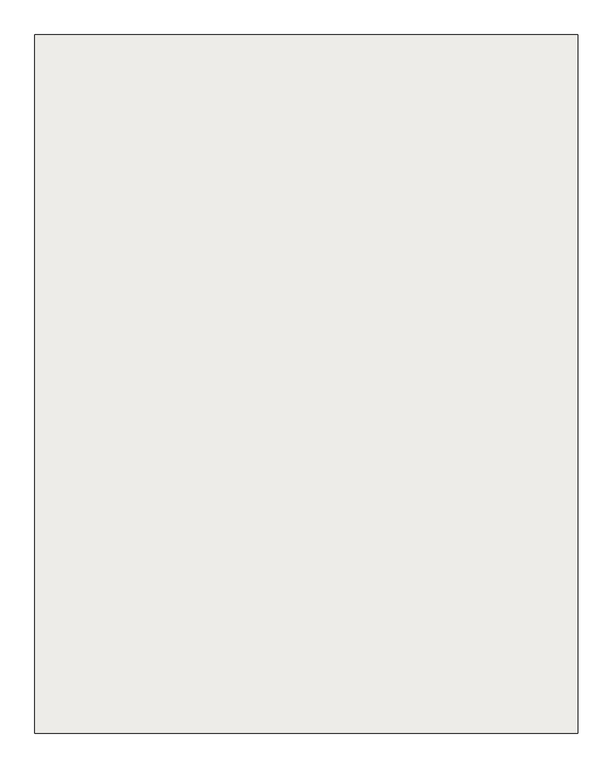
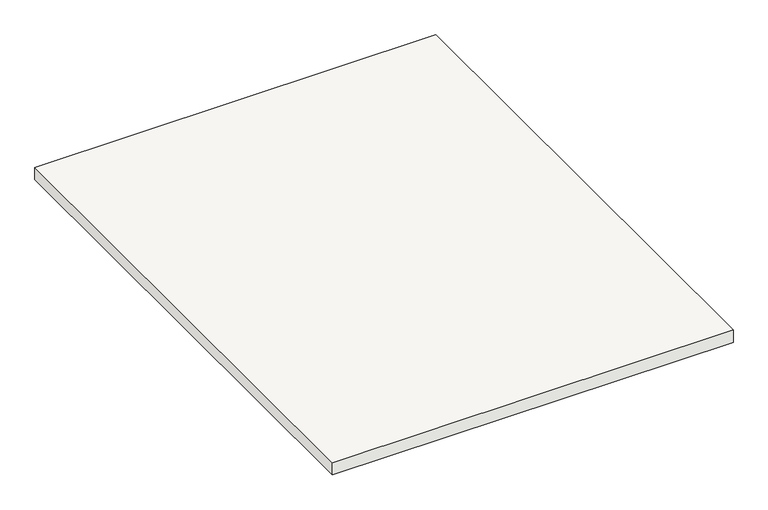
"""IFC4 building model written with IfcOpenShell, lengths in millimetres: slab geometry, Holzdecke 176 : Holzdecke 176."""

import ifcopenshell
import ifcopenshell.guid

model = None  # the IFC model being written
_history = None  # IfcOwnerHistory: only IFC2X3 demands one
_inside = {}  # id of a spatial element -> (the spatial element, [elements in it])
_under = {}  # id of a project, library or spatial element -> (it, [spatial elements below it])
_declared = {}  # id of a project -> (the project, [libraries it declares])
_typed = {}  # id of a type object -> (the type object, [elements of that type])
_made_of = {}  # id of a material, layer set ... -> (it, [elements and type objects made of it])


def new_model(schema):
    """Start an empty IFC model of exactly this schema.

    Asked for "IFC4X3", IfcOpenShell would pick the latest addendum, in which some entities
    have other attributes; the version numbers below select the first issue.
    IFC2X3 requires an IfcOwnerHistory on every rooted entity: one is made here for all.
    """
    global model, _history
    if schema == "IFC4X3":
        model = ifcopenshell.file(schema_version=(4, 3, 0, 0))
    else:
        model = ifcopenshell.file(schema=schema)
    _inside.clear()
    _under.clear()
    _declared.clear()
    _typed.clear()
    _made_of.clear()
    _history = None
    if model.schema == "IFC2X3":
        org = make("IfcOrganization", Name="unknown")
        user = make(
            "IfcPersonAndOrganization",
            ThePerson=make("IfcPerson", FamilyName="unknown"),
            TheOrganization=org,
        )
        app = make(
            "IfcApplication",
            ApplicationDeveloper=org,
            Version="unknown",
            ApplicationFullName="unknown",
            ApplicationIdentifier="unknown",
        )
        _history = make(
            "IfcOwnerHistory",
            OwningUser=user,
            OwningApplication=app,
            ChangeAction="ADDED",
            CreationDate=0,
        )
    return model


def make(cls, **values):
    """One entity of the class cls with the attributes given. An attribute that is None is left unset."""
    return model.create_entity(
        cls, **{name: value for name, value in values.items() if value is not None}
    )


def rooted(cls, **values):
    """An entity with a GlobalId (a new one), such as an element, a storey or a relation."""
    return make(cls, GlobalId=ifcopenshell.guid.new(), OwnerHistory=_history, **values)


def si_unit(unit_type, name, prefix=None):
    """IfcSIUnit, for example si_unit("LENGTHUNIT", "METRE", prefix="MILLI")."""
    return make("IfcSIUnit", UnitType=unit_type, Prefix=prefix, Name=name)


def assignment(units):
    """IfcUnitAssignment: the units of a project."""
    return None if units is None else make("IfcUnitAssignment", Units=units)


def point(xyz):
    """IfcCartesianPoint."""
    return None if xyz is None else make("IfcCartesianPoint", Coordinates=xyz)


def direction(xyz):
    """IfcDirection."""
    return None if xyz is None else make("IfcDirection", DirectionRatios=xyz)


def frame(location, z_axis=None, x_axis=None):
    """IfcAxis2Placement3D, a coordinate frame: its origin and axes. An axis left out is left unset."""
    return make(
        "IfcAxis2Placement3D",
        Location=point(location),
        Axis=direction(z_axis),
        RefDirection=direction(x_axis),
    )


def origin():
    """The frame at (0, 0, 0) with its axes left unset."""
    return frame((0.0, 0.0, 0.0))


def place(relative_to, where):
    """IfcLocalPlacement: puts the frame where relative to a parent placement (None: the world)."""
    return make(
        "IfcLocalPlacement", PlacementRelTo=relative_to, RelativePlacement=where
    )


def context(
    kind, dimensions, precision=None, world=None, true_north=None, identifier=None
):
    """IfcGeometricRepresentationContext, for example the 3D "Model" context."""
    return make(
        "IfcGeometricRepresentationContext",
        ContextIdentifier=identifier,
        ContextType=kind,
        CoordinateSpaceDimension=dimensions,
        Precision=precision,
        WorldCoordinateSystem=world,
        TrueNorth=true_north,
    )


def project(units=None, contexts=None):
    """IfcProject with its units and contexts."""
    return rooted(
        "IfcProject",
        Name="project",
        RepresentationContexts=contexts,
        UnitsInContext=assignment(units),
    )


def spatial(cls, under=None, at=None, **own):
    """A site, building, storey or space (cls), placed at a placement, below another one or the project."""
    s = rooted(cls, ObjectPlacement=at, **own)
    if under is not None:
        _under.setdefault(under.id(), (under, []))[1].append(s)
    return s


def polyline(points):
    """IfcPolyline through the points."""
    return make("IfcPolyline", Points=[point(p) for p in points])


def outline(outer, holes=None, kind="AREA"):
    """IfcArbitraryClosedProfileDef: a profile drawn as a closed curve; with holes, ...WithVoids."""
    if holes is None:
        return make("IfcArbitraryClosedProfileDef", ProfileType=kind, OuterCurve=outer)
    return make(
        "IfcArbitraryProfileDefWithVoids",
        ProfileType=kind,
        OuterCurve=outer,
        InnerCurves=holes,
    )


def extrude(swept, where, along, depth):
    """IfcExtrudedAreaSolid: the profile swept, set in the frame where, extruded along a direction by depth."""
    return make(
        "IfcExtrudedAreaSolid",
        SweptArea=swept,
        Position=where,
        ExtrudedDirection=direction(along),
        Depth=depth,
    )


def shape(context_of_items, identifier, shape_type, items):
    """IfcShapeRepresentation: the items that make up one representation, for example the "Body"."""
    return make(
        "IfcShapeRepresentation",
        ContextOfItems=context_of_items,
        RepresentationIdentifier=identifier,
        RepresentationType=shape_type,
        Items=items,
    )


def source(mapping_origin, context_of_items, identifier, shape_type, items):
    """IfcRepresentationMap: a shape defined once, which mapped items show again and again."""
    return make(
        "IfcRepresentationMap",
        MappingOrigin=mapping_origin,
        MappedRepresentation=shape(context_of_items, identifier, shape_type, items),
    )


def transform(
    local_origin,
    x_axis=None,
    y_axis=None,
    z_axis=None,
    scale=None,
    scale2=None,
    scale3=None,
    uniform=True,
):
    """IfcCartesianTransformationOperator3D, or its non-uniform kind. x_axis, y_axis, z_axis: its Axis1, 2, 3."""
    if uniform:
        return make(
            "IfcCartesianTransformationOperator3D",
            Axis1=direction(x_axis),
            Axis2=direction(y_axis),
            LocalOrigin=point(local_origin),
            Scale=scale,
            Axis3=direction(z_axis),
        )
    return make(
        "IfcCartesianTransformationOperator3DnonUniform",
        Axis1=direction(x_axis),
        Axis2=direction(y_axis),
        LocalOrigin=point(local_origin),
        Scale=scale,
        Axis3=direction(z_axis),
        Scale2=scale2,
        Scale3=scale3,
    )


def mapped(mapping_source, mapping_target):
    """IfcMappedItem: shows the shape of a source again, moved by a transform."""
    return make(
        "IfcMappedItem", MappingSource=mapping_source, MappingTarget=mapping_target
    )


def made_of(thing, what):
    """Note that an element or type object is made of a material, layer set ...; save() writes the relation."""
    if what is not None:
        _made_of.setdefault(what.id(), (what, []))[1].append(thing)
    return thing


def element(
    cls,
    number,
    at=None,
    inside=None,
    cuts=None,
    type_object=None,
    material=None,
    context=None,
    identifier="Body",
    shape_type=None,
    held_by="IfcProductDefinitionShape",
    body=None,
    shapes=None,
    **own,
):
    """One element of the class cls, such as IfcWall. Its Tag is "e" and its number.

    at: its placement. inside: the storey or other place that contains it. cuts: it is an
    opening in that element (IfcRelVoidsElement). A single representation is given by context,
    identifier, shape_type and body (its items); several are given by shapes. held_by: the class
    of the entity that holds the representations. save() writes the other relations.
    """
    e = rooted(cls, Tag="e%d" % number, ObjectPlacement=at, **own)
    if body is not None:
        shapes = [shape(context, identifier, shape_type, body)]
    if shapes is not None:
        e.Representation = make(held_by, Representations=shapes)
    if inside is not None:
        _inside.setdefault(inside.id(), (inside, []))[1].append(e)
    if cuts is not None:
        rooted(
            "IfcRelVoidsElement", RelatingBuildingElement=cuts, RelatedOpeningElement=e
        )
    if type_object is not None:
        _typed.setdefault(type_object.id(), (type_object, []))[1].append(e)
    return made_of(e, material)


def aggregate(whole, parts):
    """IfcRelAggregates: a whole, such as a stair, and the parts it consists of."""
    return rooted("IfcRelAggregates", RelatingObject=whole, RelatedObjects=parts)


def save(model, path):
    """Write the relations noted so far, then the file.

    IfcRelAggregates (storeys below a building ...), IfcRelContainedInSpatialStructure (elements
    in a storey), IfcRelDefinesByType, IfcRelAssociatesMaterial and IfcRelDeclares: one each for
    every whole, place, type object, material and project.
    """
    for whole, parts in _under.values():
        aggregate(whole, parts)
    for where, things in _inside.values():
        rooted(
            "IfcRelContainedInSpatialStructure",
            RelatedElements=things,
            RelatingStructure=where,
        )
    for kind, things in _typed.values():
        rooted("IfcRelDefinesByType", RelatedObjects=things, RelatingType=kind)
    for what, things in _made_of.values():
        rooted("IfcRelAssociatesMaterial", RelatedObjects=things, RelatingMaterial=what)
    for by, libraries in _declared.values():
        rooted("IfcRelDeclares", RelatingContext=by, RelatedDefinitions=libraries)
    model.write(path)


def slab_91406d58(model_context):
    return source(origin(), model_context, "Body", "SweptSolid", [
        extrude(outline(polyline([(15500.0, 19550.0), (15500.0, 1547.1380981), (1500.0, 1547.1380981), (1500.0, 19550.0), (15500.0, 19550.0)])), frame((0.0, 0.0, 2880.0), z_axis=(0.0, 0.0, 1.0), x_axis=(1.0, 0.0, 0.0)), (0.0, 0.0, 1.0), 450.0),
    ])


if __name__ == "__main__":
    model = new_model("IFC4")
    model_context = context("Model", 3, world=origin())
    ifc_project = project(units=[si_unit("LENGTHUNIT", "METRE", prefix="MILLI")], contexts=[model_context])
    site = spatial("IfcSite", under=ifc_project)
    building = spatial("IfcBuilding", under=site)
    placement = place(None, origin())
    slab_shape = slab_91406d58(model_context)
    element("IfcSlab", 1, ObjectType="Holzdecke 176 : Holzdecke 176", at=placement, inside=building, context=model_context, shape_type="MappedRepresentation", body=[
        mapped(slab_shape, transform((0.0, 0.0, 0.0), x_axis=(1.0, 0.0, 0.0), y_axis=(0.0, 1.0, 0.0), z_axis=(0.0, 0.0, 1.0))),
    ])
    save(model, "model.ifc")

# Revit data of these elements
# Type "Holzdecke 176 : Holzdecke 176"
#   Abrechnungsart = "m²"
#   Allright_Bauteil_ID = "0113De 0783954357"
#   Bezeichnung = "Holzdecke"
#   Codetext = "D-HOLZBALKEN1\\"
#   Gewerk = "Zimmer- und Holzbauarbeiten"
#   Material = "Holz"
#   Objektname = "Brettstapeldecke"
#   NameOverride = "Holzdecke"
#   Reference = "Holzdecke"
#   Status = "NEW"
#   PitchAngle = 0.00°
#   ThermalTransmittance = 0.0000 BTU/(h·ft²·°F)
#   2D Interaktion = yes
#   Combustible = no
#   Compartmentation = no
#   IsExternal = no
#   LoadBearing = yes
# Element 1 (IfcSlab, "Holzdecke 176 : Holzdecke 176")
#   Materials on its faces: "holzschalung"
# Materials
#   "holzschalung": class "Unassigned", colour RGB 128 128 128, transparency 0
